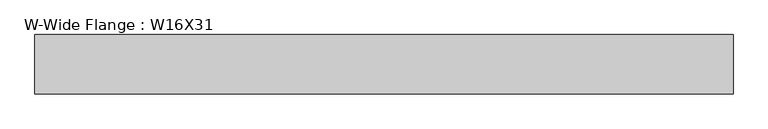
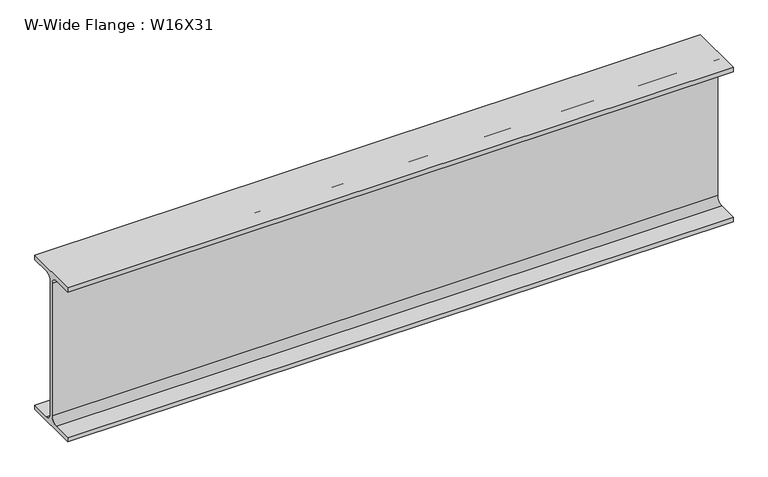
"""IFC4 building model written with IfcOpenShell, lengths in millimetres: beam geometry, W-Wide Flange : W16X31."""

from ifc_helpers import new_model, si_unit, point, frame, frame_2d, origin, place, context, project, spatial, polyline, circle_curve, trimmed, segment, composite_curve, outline, extrude, source, transform, mapped, element, save


def w_wide_flange_w16x31_e0288e10(model_context):
    return source(origin(), model_context, "Body", "SweptSolid", [
        extrude(outline(composite_curve([segment(polyline([(70.231, -190.754), (70.231, -201.93), (-70.231, -201.93), (-70.231, -190.754), (-20.8915, -190.754)]), True, "CONTINUOUS"), segment(trimmed(circle_curve(frame_2d((-20.8915, -173.355)), 17.399), [point((-20.8915, -190.754))], [point((-3.4925, -173.355))], True, "CARTESIAN"), True, "CONTINUOUS"), segment(polyline([(-3.4925, -173.355), (-3.4925, 173.355)]), True, "CONTINUOUS"), segment(trimmed(circle_curve(frame_2d((-20.8915, 173.355)), 17.399), [point((-3.4925, 173.355))], [point((-20.8915, 190.754))], True, "CARTESIAN"), True, "CONTINUOUS"), segment(polyline([(-20.8915, 190.754), (-70.231, 190.754), (-70.231, 201.93), (70.231, 201.93), (70.231, 190.754), (20.8915, 190.754)]), True, "CONTINUOUS"), segment(trimmed(circle_curve(frame_2d((20.8915, 173.355)), 17.399), [point((20.8915, 190.754))], [point((3.4925, 173.355))], True, "CARTESIAN"), True, "CONTINUOUS"), segment(polyline([(3.4925, 173.355), (3.4925, -173.355)]), True, "CONTINUOUS"), segment(trimmed(circle_curve(frame_2d((20.8915, -173.355)), 17.399), [point((3.4925, -173.355))], [point((20.8915, -190.754))], True, "CARTESIAN"), True, "CONTINUOUS"), segment(polyline([(20.8915, -190.754), (70.231, -190.754)]), True, "CONTINUOUS")], self_intersect=False)), frame((-808.6840266, 0.0, 0.0), z_axis=(1.0, 0.0, 0.0), x_axis=(0.0, 1.0, 0.0)), (0.0, 0.0, 1.0), 1649.3265072),
    ])


if __name__ == "__main__":
    model = new_model("IFC4")
    model_context = context("Model", 3, world=origin())
    ifc_project = project(units=[si_unit("LENGTHUNIT", "METRE", prefix="MILLI")], contexts=[model_context])
    site = spatial("IfcSite", under=ifc_project)
    building = spatial("IfcBuilding", under=site)
    placement = place(None, origin())
    w_wide_flange_w16x31_shape = w_wide_flange_w16x31_e0288e10(model_context)
    element("IfcBeam", 1, ObjectType="W-Wide Flange : W16X31", at=placement, inside=building, context=model_context, shape_type="MappedRepresentation", body=[
        mapped(w_wide_flange_w16x31_shape, transform((0.0, 0.0, 0.0), x_axis=(1.0, 0.0, 0.0), y_axis=(0.0, 1.0, 0.0), z_axis=(0.0, 0.0, 1.0))),
    ])
    save(model, "model.ifc")

# Revit data of these elements
# Type "W-Wide Flange : W16X31"
#   Assembly Code = "B10"
#   W = 31
#   Start Extension Calculation [instance default] = 10' - 0"
#   Start Extension [instance default] = -0' - 0 1/2"
#   End Extension Calculation [instance default] = 10' - 0"
#   End Extension [instance default] = -0' - 0 1/2"
#   Length [instance default] = 5' - 0"
#   bf = 0' - 5.53"
#   d = 1' - 3.9"
#   k = 0' - 1 1/8"
#   k2 = 0' - 0.685"
#   tf = 0' - 0.44"
#   tw = 0' - 0.275"
#   A = 0.0634028 SF
#   Beam Material [instance default] = Metal - Steel - ASTM A992
# Element 1 (IfcBeam, "W-Wide Flange : W16X31")
#   Materials on its faces: "Metal - Steel - ASTM A992"
# Materials
#   "Metal - Steel - ASTM A992": class "Metal", colour RGB 128 0 0, transparency 0
